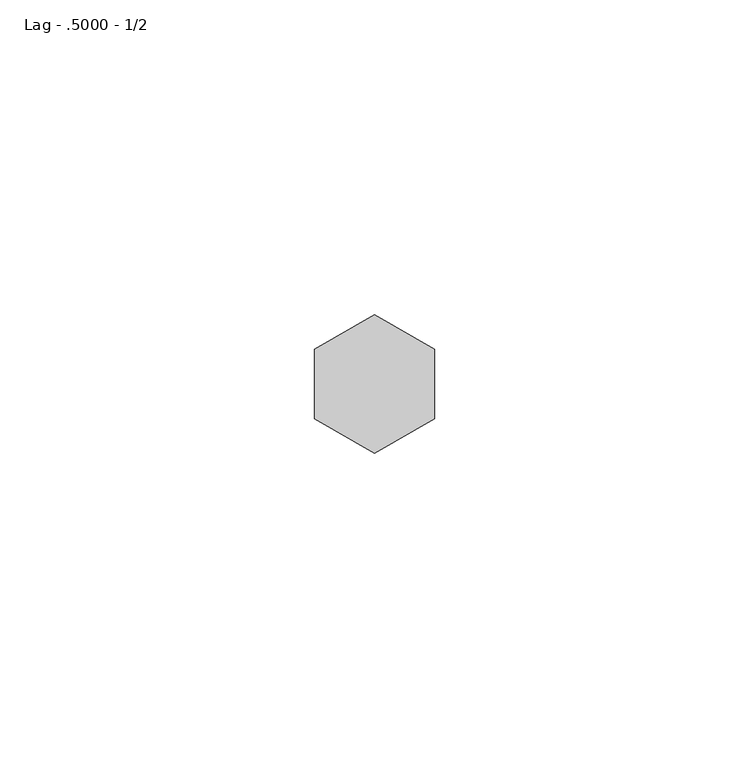
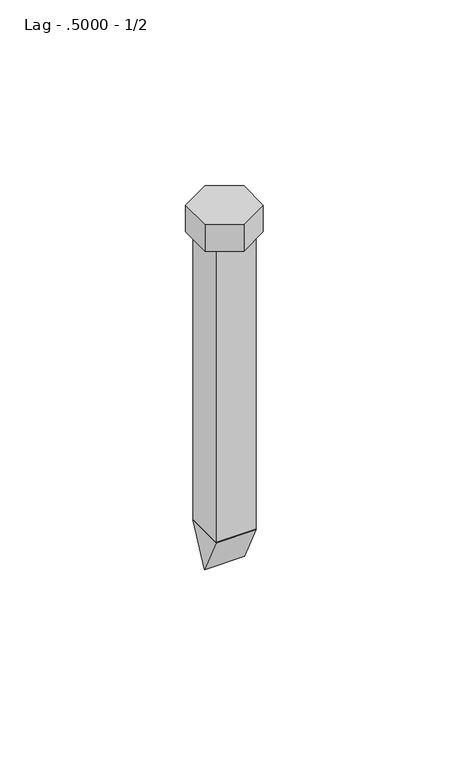
"""IFC4 building model written with IfcOpenShell, lengths in millimetres: fastener geometry, 060523 - W_P_C - Fastenings - Generic - SQUARE : Lag - .5000 - 1/2."""

import ifcopenshell
import ifcopenshell.guid

model = None  # the IFC model being written
_history = None  # IfcOwnerHistory: only IFC2X3 demands one
_inside = {}  # id of a spatial element -> (the spatial element, [elements in it])
_under = {}  # id of a project, library or spatial element -> (it, [spatial elements below it])
_declared = {}  # id of a project -> (the project, [libraries it declares])
_typed = {}  # id of a type object -> (the type object, [elements of that type])
_made_of = {}  # id of a material, layer set ... -> (it, [elements and type objects made of it])


def new_model(schema):
    """Start an empty IFC model of exactly this schema.

    Asked for "IFC4X3", IfcOpenShell would pick the latest addendum, in which some entities
    have other attributes; the version numbers below select the first issue.
    IFC2X3 requires an IfcOwnerHistory on every rooted entity: one is made here for all.
    """
    global model, _history
    if schema == "IFC4X3":
        model = ifcopenshell.file(schema_version=(4, 3, 0, 0))
    else:
        model = ifcopenshell.file(schema=schema)
    _inside.clear()
    _under.clear()
    _declared.clear()
    _typed.clear()
    _made_of.clear()
    _history = None
    if model.schema == "IFC2X3":
        org = make("IfcOrganization", Name="unknown")
        user = make(
            "IfcPersonAndOrganization",
            ThePerson=make("IfcPerson", FamilyName="unknown"),
            TheOrganization=org,
        )
        app = make(
            "IfcApplication",
            ApplicationDeveloper=org,
            Version="unknown",
            ApplicationFullName="unknown",
            ApplicationIdentifier="unknown",
        )
        _history = make(
            "IfcOwnerHistory",
            OwningUser=user,
            OwningApplication=app,
            ChangeAction="ADDED",
            CreationDate=0,
        )
    return model


def make(cls, **values):
    """One entity of the class cls with the attributes given. An attribute that is None is left unset."""
    return model.create_entity(
        cls, **{name: value for name, value in values.items() if value is not None}
    )


def rooted(cls, **values):
    """An entity with a GlobalId (a new one), such as an element, a storey or a relation."""
    return make(cls, GlobalId=ifcopenshell.guid.new(), OwnerHistory=_history, **values)


def si_unit(unit_type, name, prefix=None):
    """IfcSIUnit, for example si_unit("LENGTHUNIT", "METRE", prefix="MILLI")."""
    return make("IfcSIUnit", UnitType=unit_type, Prefix=prefix, Name=name)


def assignment(units):
    """IfcUnitAssignment: the units of a project."""
    return None if units is None else make("IfcUnitAssignment", Units=units)


def point(xyz):
    """IfcCartesianPoint."""
    return None if xyz is None else make("IfcCartesianPoint", Coordinates=xyz)


def direction(xyz):
    """IfcDirection."""
    return None if xyz is None else make("IfcDirection", DirectionRatios=xyz)


def frame(location, z_axis=None, x_axis=None):
    """IfcAxis2Placement3D, a coordinate frame: its origin and axes. An axis left out is left unset."""
    return make(
        "IfcAxis2Placement3D",
        Location=point(location),
        Axis=direction(z_axis),
        RefDirection=direction(x_axis),
    )


def origin():
    """The frame at (0, 0, 0) with its axes left unset."""
    return frame((0.0, 0.0, 0.0))


def origin_with_axes():
    """The frame at (0, 0, 0) with the z axis (0, 0, 1) and the x axis (1, 0, 0) written out."""
    return frame((0.0, 0.0, 0.0), z_axis=(0.0, 0.0, 1.0), x_axis=(1.0, 0.0, 0.0))


def place(relative_to, where):
    """IfcLocalPlacement: puts the frame where relative to a parent placement (None: the world)."""
    return make(
        "IfcLocalPlacement", PlacementRelTo=relative_to, RelativePlacement=where
    )


def context(
    kind, dimensions, precision=None, world=None, true_north=None, identifier=None
):
    """IfcGeometricRepresentationContext, for example the 3D "Model" context."""
    return make(
        "IfcGeometricRepresentationContext",
        ContextIdentifier=identifier,
        ContextType=kind,
        CoordinateSpaceDimension=dimensions,
        Precision=precision,
        WorldCoordinateSystem=world,
        TrueNorth=true_north,
    )


def project(units=None, contexts=None):
    """IfcProject with its units and contexts."""
    return rooted(
        "IfcProject",
        Name="project",
        RepresentationContexts=contexts,
        UnitsInContext=assignment(units),
    )


def spatial(cls, under=None, at=None, **own):
    """A site, building, storey or space (cls), placed at a placement, below another one or the project."""
    s = rooted(cls, ObjectPlacement=at, **own)
    if under is not None:
        _under.setdefault(under.id(), (under, []))[1].append(s)
    return s


def polyline(points):
    """IfcPolyline through the points."""
    return make("IfcPolyline", Points=[point(p) for p in points])


def outline(outer, holes=None, kind="AREA"):
    """IfcArbitraryClosedProfileDef: a profile drawn as a closed curve; with holes, ...WithVoids."""
    if holes is None:
        return make("IfcArbitraryClosedProfileDef", ProfileType=kind, OuterCurve=outer)
    return make(
        "IfcArbitraryProfileDefWithVoids",
        ProfileType=kind,
        OuterCurve=outer,
        InnerCurves=holes,
    )


def extrude(swept, where, along, depth):
    """IfcExtrudedAreaSolid: the profile swept, set in the frame where, extruded along a direction by depth."""
    return make(
        "IfcExtrudedAreaSolid",
        SweptArea=swept,
        Position=where,
        ExtrudedDirection=direction(along),
        Depth=depth,
    )


def shape(context_of_items, identifier, shape_type, items):
    """IfcShapeRepresentation: the items that make up one representation, for example the "Body"."""
    return make(
        "IfcShapeRepresentation",
        ContextOfItems=context_of_items,
        RepresentationIdentifier=identifier,
        RepresentationType=shape_type,
        Items=items,
    )


def source(mapping_origin, context_of_items, identifier, shape_type, items):
    """IfcRepresentationMap: a shape defined once, which mapped items show again and again."""
    return make(
        "IfcRepresentationMap",
        MappingOrigin=mapping_origin,
        MappedRepresentation=shape(context_of_items, identifier, shape_type, items),
    )


def transform(
    local_origin,
    x_axis=None,
    y_axis=None,
    z_axis=None,
    scale=None,
    scale2=None,
    scale3=None,
    uniform=True,
):
    """IfcCartesianTransformationOperator3D, or its non-uniform kind. x_axis, y_axis, z_axis: its Axis1, 2, 3."""
    if uniform:
        return make(
            "IfcCartesianTransformationOperator3D",
            Axis1=direction(x_axis),
            Axis2=direction(y_axis),
            LocalOrigin=point(local_origin),
            Scale=scale,
            Axis3=direction(z_axis),
        )
    return make(
        "IfcCartesianTransformationOperator3DnonUniform",
        Axis1=direction(x_axis),
        Axis2=direction(y_axis),
        LocalOrigin=point(local_origin),
        Scale=scale,
        Axis3=direction(z_axis),
        Scale2=scale2,
        Scale3=scale3,
    )


def mapped(mapping_source, mapping_target):
    """IfcMappedItem: shows the shape of a source again, moved by a transform."""
    return make(
        "IfcMappedItem", MappingSource=mapping_source, MappingTarget=mapping_target
    )


def made_of(thing, what):
    """Note that an element or type object is made of a material, layer set ...; save() writes the relation."""
    if what is not None:
        _made_of.setdefault(what.id(), (what, []))[1].append(thing)
    return thing


def element(
    cls,
    number,
    at=None,
    inside=None,
    cuts=None,
    type_object=None,
    material=None,
    context=None,
    identifier="Body",
    shape_type=None,
    held_by="IfcProductDefinitionShape",
    body=None,
    shapes=None,
    **own,
):
    """One element of the class cls, such as IfcWall. Its Tag is "e" and its number.

    at: its placement. inside: the storey or other place that contains it. cuts: it is an
    opening in that element (IfcRelVoidsElement). A single representation is given by context,
    identifier, shape_type and body (its items); several are given by shapes. held_by: the class
    of the entity that holds the representations. save() writes the other relations.
    """
    e = rooted(cls, Tag="e%d" % number, ObjectPlacement=at, **own)
    if body is not None:
        shapes = [shape(context, identifier, shape_type, body)]
    if shapes is not None:
        e.Representation = make(held_by, Representations=shapes)
    if inside is not None:
        _inside.setdefault(inside.id(), (inside, []))[1].append(e)
    if cuts is not None:
        rooted(
            "IfcRelVoidsElement", RelatingBuildingElement=cuts, RelatedOpeningElement=e
        )
    if type_object is not None:
        _typed.setdefault(type_object.id(), (type_object, []))[1].append(e)
    return made_of(e, material)


def aggregate(whole, parts):
    """IfcRelAggregates: a whole, such as a stair, and the parts it consists of."""
    return rooted("IfcRelAggregates", RelatingObject=whole, RelatedObjects=parts)


def save(model, path):
    """Write the relations noted so far, then the file.

    IfcRelAggregates (storeys below a building ...), IfcRelContainedInSpatialStructure (elements
    in a storey), IfcRelDefinesByType, IfcRelAssociatesMaterial and IfcRelDeclares: one each for
    every whole, place, type object, material and project.
    """
    for whole, parts in _under.values():
        aggregate(whole, parts)
    for where, things in _inside.values():
        rooted(
            "IfcRelContainedInSpatialStructure",
            RelatedElements=things,
            RelatingStructure=where,
        )
    for kind, things in _typed.values():
        rooted("IfcRelDefinesByType", RelatedObjects=things, RelatingType=kind)
    for what, things in _made_of.values():
        rooted("IfcRelAssociatesMaterial", RelatedObjects=things, RelatingMaterial=what)
    for by, libraries in _declared.values():
        rooted("IfcRelDeclares", RelatingContext=by, RelatedDefinitions=libraries)
    model.write(path)


def lag_5000_1_2_34a09ce3(model_context):
    return source(origin(), model_context, "Body", "SweptSolid", [
        extrude(outline(polyline([(0.0, -114.696875), (-6.5484375, -101.6), (6.5484375, -101.6), (0.0, -114.696875)])), frame((-6.5484375, 0.0, 0.0), z_axis=(1.0, 0.0, 0.0), x_axis=(0.0, 1.0, 0.0)), (0.0, 0.0, 1.0), 13.096875),
        extrude(outline(polyline([(-9.525, 5.4992613), (0.0, 10.9985226), (9.525, 5.4992613), (9.525, -5.4992613), (0.0, -10.9985226), (-9.525, -5.4992613), (-9.525, 5.4992613)])), origin_with_axes(), (0.0, 0.0, 1.0), 9.2273437),
        extrude(outline(polyline([(-6.5484375, 6.5484375), (6.5484375, 6.5484375), (6.5484375, -6.5484375), (-6.5484375, -6.5484375), (-6.5484375, 6.5484375)])), frame((0.0, 0.0, -101.6), z_axis=(0.0, 0.0, 1.0), x_axis=(1.0, 0.0, 0.0)), (0.0, 0.0, 1.0), 101.6),
    ])


if __name__ == "__main__":
    model = new_model("IFC4")
    model_context = context("Model", 3, world=origin())
    ifc_project = project(units=[si_unit("LENGTHUNIT", "METRE", prefix="MILLI")], contexts=[model_context])
    site = spatial("IfcSite", under=ifc_project)
    building = spatial("IfcBuilding", under=site)
    placement = place(None, origin())
    lag_5000_1_2_shape = lag_5000_1_2_34a09ce3(model_context)
    element("IfcFastener", 1, ObjectType="060523 - W_P_C - Fastenings - Generic - SQUARE : Lag - .5000 - 1/2", at=placement, inside=building, context=model_context, shape_type="MappedRepresentation", body=[
        mapped(lag_5000_1_2_shape, transform((0.0, 0.0, 0.0), x_axis=(1.0, 0.0, 0.0), y_axis=(0.0, 1.0, 0.0), z_axis=(0.0, 0.0, 1.0))),
    ])
    save(model, "model.ifc")

# Revit data of these elements
# Type "060523 - W_P_C - Fastenings - Generic - SQUARE : Lag - .5000 - 1/2"
#   Washer_Thickness = 0' - 0 31/256"
#   Washer Radius = 0' - 0 159/256"
#   Washer Offset - Head = 0' - 0"
#   Washer Offset = 0' - 0"
#   Thickness_of_Substrate [instance default] = 0' - 1"
#   Side = 0' - 0 111/256"
#   Radius = 0' - 0 33/128"
#   Length [instance default] = 0' - 4"
#   Head Size = 0' - 0 3/4"
#   Head Radius = 0' - 0 3/8"
#   Head Height = 0' - 0 93/256"
#   Double Diameter = 0' - 1 1/32"
#   Diameter = 0' - 0 33/64"
#   Default Elevation = 4' - 0"
#   Washer_Nut_Visibility = no
#   Washer_Head_Visibility = no
#   Round_Head_Visibility = no
#   Point Visibility = yes
#   Nut_Visibility = no
#   Hex_Head_Visiblilty = yes
#   Washer Material = none
#   Bolt Material (Size) = AT SILL - FASTENER AT 24" O.C.
# Element 1 (IfcFastener, "060523 - W_P_C - Fastenings - Generic - SQUARE : Lag - .5000 - 1/2")
#   Materials on its faces: "AT SILL - FASTENER AT 24\" O.C."
# Materials
#   "AT SILL - FASTENER AT 24\" O.C.": class "Generic", colour RGB 120 120 120, transparency 0, Cost = 0
